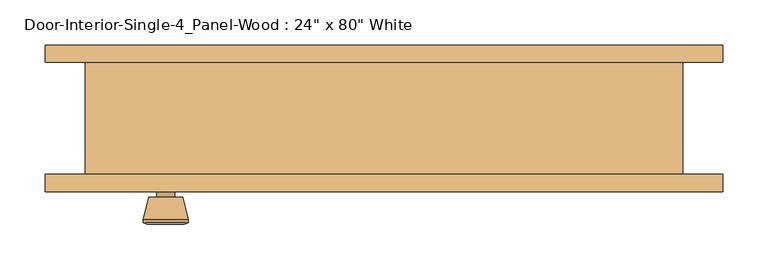
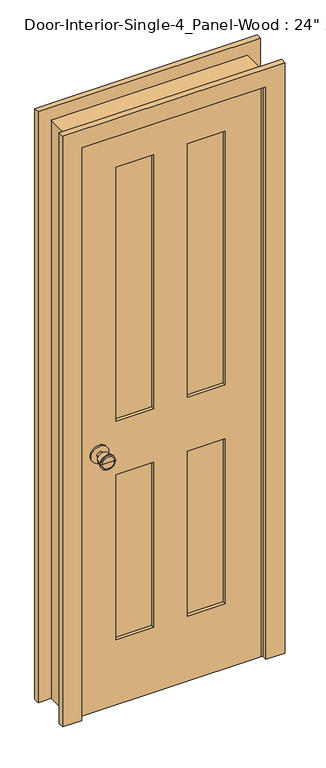
"""IFC4 building model written with IfcOpenShell, lengths in millimetres: door geometry."""

from ifc_helpers import new_model, si_unit, point, frame, frame_2d, origin, place, context, project, spatial, polyline, circle_curve, trimmed, segment, composite_curve, outline, extrude, faceted_brep, source, transform, mapped, element, save
from ifc_brep_helpers import plane_surface, cylinder_surface, revolved_surface, advanced_brep


def door_cd006500(model_context):
    return source(origin(), model_context, "Body", "SolidModel", [
        advanced_brep(
        [(-241.3, -17.8125, 914.4), (-251.3, -17.8125, 914.4), (-231.3, -17.8125, 914.4), (-220.8241324, 31.1875, 914.4), (-261.7758676, 31.1875, 914.4), (-241.3, 31.1875, 914.4), (-216.3, 29.3596319, 914.4), (-266.3, 29.3596319, 914.4), (-216.3, 25.8959537, 914.4), (-266.3, 25.8959537, 914.4), (-222.663764, 1.1875, 914.4), (-259.936236, 1.1875, 914.4), (-231.3, 1.1875, 914.4), (-251.3, 1.1875, 914.4)],
        [
            (0, 1),
            (1, 2, circle_curve(frame((-241.3, -17.8125, 914.4), z_axis=(0.0, -1.0, 0.0), x_axis=(-1.0, 0.0, 0.0)), 10.0)),
            (2, 0),
            (2, 1, circle_curve(frame((-241.3, -17.8125, 914.4), z_axis=(0.0, -1.0, 0.0), x_axis=(-1.0, 0.0, 0.0)), 10.0)),
            (3, 4, circle_curve(frame((-241.3, 31.1875, 914.4), z_axis=(0.0, 1.0, 0.0), x_axis=(-1.0, 0.0, 0.0)), 20.4758676)),
            (4, 5),
            (5, 3),
            (4, 3, circle_curve(frame((-241.3, 31.1875, 914.4), z_axis=(0.0, 1.0, 0.0), x_axis=(-1.0, 0.0, 0.0)), 20.4758676)),
            (6, 7, circle_curve(frame((-241.3, 29.3596319, 914.4), z_axis=(0.0, 1.0, 0.0), x_axis=(-1.0, 0.0, 0.0)), 25.0)),
            (7, 4),
            (3, 6),
            (7, 6, circle_curve(frame((-241.3, 29.3596319, 914.4), z_axis=(0.0, 1.0, 0.0), x_axis=(-1.0, 0.0, 0.0)), 25.0)),
            (8, 9, circle_curve(frame((-241.3, 25.8959537, 914.4), z_axis=(0.0, 1.0, 0.0), x_axis=(-1.0, 0.0, 0.0)), 25.0)),
            (9, 7),
            (6, 8),
            (9, 8, circle_curve(frame((-241.3, 25.8959537, 914.4), z_axis=(0.0, 1.0, 0.0), x_axis=(-1.0, 0.0, 0.0)), 25.0)),
            (10, 11, circle_curve(frame((-241.3, 1.1875, 914.4), z_axis=(0.0, 1.0, 0.0), x_axis=(-1.0, 0.0, 0.0)), 18.636236)),
            (11, 9),
            (8, 10),
            (11, 10, circle_curve(frame((-241.3, 1.1875, 914.4), z_axis=(0.0, 1.0, 0.0), x_axis=(-1.0, 0.0, 0.0)), 18.636236)),
            (12, 13, circle_curve(frame((-241.3, 1.1875, 914.4), z_axis=(0.0, 1.0, 0.0), x_axis=(-1.0, 0.0, 0.0)), 10.0)),
            (13, 11),
            (10, 12),
            (13, 12, circle_curve(frame((-241.3, 1.1875, 914.4), z_axis=(0.0, 1.0, 0.0), x_axis=(-1.0, 0.0, 0.0)), 10.0)),
            (1, 13),
            (12, 2),
        ],
        [
            plane_surface(frame((-241.3, -17.8125, 914.4), z_axis=(0.0, -1.0, 0.0), x_axis=(-1.0, 0.0, 0.0))),
            plane_surface(frame((-241.3, 31.1875, 914.4), z_axis=(0.0, 1.0, 0.0), x_axis=(-1.0, 0.0, 0.0))),
            revolved_surface(polyline([(-261.7758676, 31.1875, 914.4), (-266.3, 29.3596319, 914.4)]), (-241.3, -17.8125, 914.4), (0.0, -1.0, 0.0)),
            cylinder_surface(frame((-241.3, -17.8125, 914.4), z_axis=(0.0, -1.0, 0.0), x_axis=(-1.0, 0.0, 0.0)), 25.0),
            revolved_surface(polyline([(-266.3, 25.8959537, 914.4), (-259.936236, 1.1875, 914.4)]), (-241.3, -17.8125, 914.4), (0.0, -1.0, 0.0)),
            plane_surface(frame((-241.3, 1.1875, 914.4), z_axis=(0.0, -1.0, 0.0), x_axis=(-1.0, 0.0, 0.0))),
            cylinder_surface(frame((-241.3, -17.8125, 914.4), z_axis=(0.0, -1.0, 0.0), x_axis=(-1.0, 0.0, 0.0)), 10.0),
        ],
        [
            (0, [[1, 2, 3]]),
            (0, [[-3, 4, -1]]),
            (1, [[5, 6, 7]]),
            (1, [[8, -7, -6]]),
            (2, [[9, 10, -5, 11]]),
            (2, [[12, -11, -8, -10]]),
            (3, [[13, 14, -9, 15]]),
            (3, [[16, -15, -12, -14]]),
            (4, [[17, 18, -13, 19]]),
            (4, [[20, -19, -16, -18]]),
            (5, [[21, 22, -17, 23]]),
            (5, [[24, -23, -20, -22]]),
            (6, [[-2, 25, -21, 26]]),
            (6, [[-4, -26, -24, -25]]),
        ],
    ),
        extrude(outline(composite_curve([segment(trimmed(circle_curve(frame_2d((914.4, -241.3)), 30.0), [point((914.4, -271.3))], [point((914.4, -211.3))], False, "CARTESIAN"), True, "CONTINUOUS"), segment(trimmed(circle_curve(frame_2d((914.4, -241.3)), 30.0), [point((914.4, -211.3))], [point((914.4, -271.3))], False, "CARTESIAN"), True, "CONTINUOUS")], self_intersect=False)), frame((0.0, -23.8125, 0.0), z_axis=(0.0, 1.0, 0.0), x_axis=(0.0, 0.0, 1.0)), (0.0, 0.0, 1.0), 6.0),
        advanced_brep(
        [(-241.3, -64.7375, 914.4), (-231.3, -64.7375, 914.4), (-251.3, -64.7375, 914.4), (-220.8241324, -113.7375, 914.4), (-241.3, -113.7375, 914.4), (-261.7758676, -113.7375, 914.4), (-216.3, -111.9096319, 914.4), (-266.3, -111.9096319, 914.4), (-216.3, -108.4459537, 914.4), (-266.3, -108.4459537, 914.4), (-222.663764, -83.7375, 914.4), (-259.936236, -83.7375, 914.4), (-231.3, -83.7375, 914.4), (-251.3, -83.7375, 914.4)],
        [
            (0, 1),
            (1, 2, circle_curve(frame((-241.3, -64.7375, 914.4), z_axis=(0.0, 1.0, 0.0), x_axis=(-1.0, 0.0, 0.0)), 10.0)),
            (2, 0),
            (2, 1, circle_curve(frame((-241.3, -64.7375, 914.4), z_axis=(0.0, 1.0, 0.0), x_axis=(-1.0, 0.0, 0.0)), 10.0)),
            (3, 4),
            (4, 5),
            (5, 3, circle_curve(frame((-241.3, -113.7375, 914.4), z_axis=(0.0, -1.0, 0.0), x_axis=(-1.0, 0.0, 0.0)), 20.4758676)),
            (3, 5, circle_curve(frame((-241.3, -113.7375, 914.4), z_axis=(0.0, -1.0, 0.0), x_axis=(-1.0, 0.0, 0.0)), 20.4758676)),
            (6, 3),
            (5, 7),
            (7, 6, circle_curve(frame((-241.3, -111.9096319, 914.4), z_axis=(0.0, -1.0, 0.0), x_axis=(-1.0, 0.0, 0.0)), 25.0)),
            (6, 7, circle_curve(frame((-241.3, -111.9096319, 914.4), z_axis=(0.0, -1.0, 0.0), x_axis=(-1.0, 0.0, 0.0)), 25.0)),
            (8, 6),
            (7, 9),
            (9, 8, circle_curve(frame((-241.3, -108.4459537, 914.4), z_axis=(0.0, -1.0, 0.0), x_axis=(-1.0, 0.0, 0.0)), 25.0)),
            (8, 9, circle_curve(frame((-241.3, -108.4459537, 914.4), z_axis=(0.0, -1.0, 0.0), x_axis=(-1.0, 0.0, 0.0)), 25.0)),
            (10, 8),
            (9, 11),
            (11, 10, circle_curve(frame((-241.3, -83.7375, 914.4), z_axis=(0.0, -1.0, 0.0), x_axis=(-1.0, 0.0, 0.0)), 18.636236)),
            (10, 11, circle_curve(frame((-241.3, -83.7375, 914.4), z_axis=(0.0, -1.0, 0.0), x_axis=(-1.0, 0.0, 0.0)), 18.636236)),
            (12, 10),
            (11, 13),
            (13, 12, circle_curve(frame((-241.3, -83.7375, 914.4), z_axis=(0.0, -1.0, 0.0), x_axis=(-1.0, 0.0, 0.0)), 10.0)),
            (12, 13, circle_curve(frame((-241.3, -83.7375, 914.4), z_axis=(0.0, -1.0, 0.0), x_axis=(-1.0, 0.0, 0.0)), 10.0)),
            (1, 12),
            (13, 2),
        ],
        [
            plane_surface(frame((-241.3, -64.7375, 914.4), z_axis=(0.0, 1.0, 0.0), x_axis=(-1.0, 0.0, 0.0))),
            plane_surface(frame((-241.3, -113.7375, 914.4), z_axis=(0.0, -1.0, 0.0), x_axis=(-1.0, 0.0, 0.0))),
            revolved_surface(polyline([(-261.7758676, -113.7375, 914.4), (-266.3, -111.9096319, 914.4)]), (-241.3, -64.7375, 914.4), (0.0, 1.0, 0.0)),
            cylinder_surface(frame((-241.3, -64.7375, 914.4), z_axis=(0.0, 1.0, 0.0), x_axis=(-1.0, 0.0, 0.0)), 25.0),
            revolved_surface(polyline([(-266.3, -108.4459537, 914.4), (-259.936236, -83.7375, 914.4)]), (-241.3, -64.7375, 914.4), (0.0, 1.0, 0.0)),
            plane_surface(frame((-241.3, -83.7375, 914.4), z_axis=(0.0, 1.0, 0.0), x_axis=(-1.0, 0.0, 0.0))),
            cylinder_surface(frame((-241.3, -64.7375, 914.4), z_axis=(0.0, 1.0, 0.0), x_axis=(-1.0, 0.0, 0.0)), 10.0),
        ],
        [
            (0, [[1, 2, 3]]),
            (0, [[-3, 4, -1]]),
            (1, [[5, 6, 7]]),
            (1, [[-6, -5, 8]]),
            (2, [[9, -7, 10, 11]]),
            (2, [[-10, -8, -9, 12]]),
            (3, [[13, -11, 14, 15]]),
            (3, [[-14, -12, -13, 16]]),
            (4, [[17, -15, 18, 19]]),
            (4, [[-18, -16, -17, 20]]),
            (5, [[21, -19, 22, 23]]),
            (5, [[-22, -20, -21, 24]]),
            (6, [[25, -23, 26, -2]]),
            (6, [[-26, -24, -25, -4]]),
        ],
    ),
        extrude(outline(composite_curve([segment(trimmed(circle_curve(frame_2d((914.4, -241.3)), 30.0), [point((914.4, -271.3))], [point((914.4, -211.3))], False, "CARTESIAN"), True, "CONTINUOUS"), segment(trimmed(circle_curve(frame_2d((914.4, -241.3)), 30.0), [point((914.4, -211.3))], [point((914.4, -271.3))], False, "CARTESIAN"), True, "CONTINUOUS")], self_intersect=False)), frame((0.0, -64.7375, 0.0), z_axis=(0.0, 1.0, 0.0), x_axis=(0.0, 0.0, 1.0)), (0.0, 0.0, 1.0), 6.0),
        extrude(outline(polyline([(184.15, -35.4541667), (184.15, -47.0958333), (57.15, -47.0958333), (57.15, -35.4541667), (184.15, -35.4541667)])), frame((0.0, 0.0, 1009.65), z_axis=(0.0, 0.0, 1.0), x_axis=(1.0, 0.0, 0.0)), (0.0, 0.0, 1.0), 903.2875),
        extrude(outline(polyline([(-57.15, -35.4541667), (-57.15, -47.0958333), (-184.15, -47.0958333), (-184.15, -35.4541667), (-57.15, -35.4541667)])), frame((0.0, 0.0, 1009.65), z_axis=(0.0, 0.0, 1.0), x_axis=(1.0, 0.0, 0.0)), (0.0, 0.0, 1.0), 903.2875),
        extrude(outline(polyline([(184.15, -35.4541667), (184.15, -47.0958333), (57.15, -47.0958333), (57.15, -35.4541667), (184.15, -35.4541667)])), frame((0.0, 0.0, 231.775), z_axis=(0.0, 0.0, 1.0), x_axis=(1.0, 0.0, 0.0)), (0.0, 0.0, 1.0), 587.375),
        extrude(outline(polyline([(-57.15, -35.4541667), (-57.15, -47.0958333), (-184.15, -47.0958333), (-184.15, -35.4541667), (-57.15, -35.4541667)])), frame((0.0, 0.0, 231.775), z_axis=(0.0, 0.0, 1.0), x_axis=(1.0, 0.0, 0.0)), (0.0, 0.0, 1.0), 587.375),
        extrude(outline(polyline([(2032.0, -304.8), (0.0, -304.8), (0.0, 304.8), (2032.0, 304.8), (2032.0, -304.8)]), holes=[polyline([(1912.9375, 57.15), (1912.9375, 184.15), (1009.65, 184.15), (1009.65, 57.15), (1912.9375, 57.15)]), polyline([(1009.65, -57.15), (1009.65, -184.15), (1912.9375, -184.15), (1912.9375, -57.15), (1009.65, -57.15)]), polyline([(819.15, 57.15), (819.15, 184.15), (231.775, 184.15), (231.775, 57.15), (819.15, 57.15)]), polyline([(231.775, -57.15), (231.775, -184.15), (819.15, -184.15), (819.15, -57.15), (231.775, -57.15)])]), frame((0.0, -58.7375, 0.0), z_axis=(0.0, 1.0, 0.0), x_axis=(0.0, 0.0, 1.0)), (0.0, 0.0, 1.0), 34.925),
        faceted_brep([(330.2, -58.7375, 0.0), (304.8, -58.7375, 0.0), (304.8, -23.8125, 0.0), (292.1, -23.8125, 0.0), (292.1, 11.1125, 0.0), (304.8, 11.1125, 0.0), (304.8, 65.0875, 0.0), (330.2, 65.0875, 0.0), (330.2, 65.0875, 2057.4), (330.2, -58.7375, 2057.4), (304.8, 65.0875, 2032.0), (-304.8, 65.0875, 2032.0), (-304.8, 65.0875, 0.0), (-330.2, 65.0875, 0.0), (-330.2, 65.0875, 2057.4), (304.8, 11.1125, 2032.0), (292.1, 11.1125, 2019.3), (-292.1, 11.1125, 2019.3), (-292.1, 11.1125, 0.0), (-304.8, 11.1125, 0.0), (-304.8, 11.1125, 2032.0), (292.1, -23.8125, 2019.3), (304.8, -23.8125, 2032.0), (-304.8, -23.8125, 2032.0), (-304.8, -23.8125, 0.0), (-292.1, -23.8125, 0.0), (-292.1, -23.8125, 2019.3), (304.8, -58.7375, 2032.0), (-330.2, -58.7375, 2057.4), (-330.2, -58.7375, 0.0), (-304.8, -58.7375, 0.0), (-304.8, -58.7375, 2032.0)], [[[0, 1, 2, 3, 4, 5, 6, 7]], [[7, 8, 9, 0]], [[6, 10, 11, 12, 13, 14, 8, 7]], [[5, 15, 10, 6]], [[4, 16, 17, 18, 19, 20, 15, 5]], [[3, 21, 16, 4]], [[2, 22, 23, 24, 25, 26, 21, 3]], [[1, 27, 22, 2]], [[0, 9, 28, 29, 30, 31, 27, 1]], [[8, 14, 28, 9]], [[15, 20, 11, 10]], [[21, 26, 17, 16]], [[27, 31, 23, 22]], [[29, 13, 12, 19, 18, 25, 24, 30]], [[14, 13, 29, 28]], [[20, 19, 12, 11]], [[26, 25, 18, 17]], [[31, 30, 24, 23]]]),
        extrude(outline(polyline([(0.0, 374.65), (2101.85, 374.65), (2101.85, -374.65), (0.0, -374.65), (0.0, -311.15), (2038.35, -311.15), (2038.35, 311.15), (0.0, 311.15), (0.0, 374.65)])), frame((0.0, 65.0875, 0.0), z_axis=(0.0, 1.0, 0.0), x_axis=(0.0, 0.0, 1.0)), (0.0, 0.0, 1.0), 19.05),
        extrude(outline(polyline([(0.0, 374.65), (2101.85, 374.65), (2101.85, -374.65), (0.0, -374.65), (0.0, -311.15), (2038.35, -311.15), (2038.35, 311.15), (0.0, 311.15), (0.0, 374.65)])), frame((0.0, -77.7875, 0.0), z_axis=(0.0, 1.0, 0.0), x_axis=(0.0, 0.0, 1.0)), (0.0, 0.0, 1.0), 19.05),
    ])


if __name__ == "__main__":
    model = new_model("IFC4")
    model_context = context("Model", 3, world=origin())
    ifc_project = project(units=[si_unit("LENGTHUNIT", "METRE", prefix="MILLI")], contexts=[model_context])
    site = spatial("IfcSite", under=ifc_project)
    building = spatial("IfcBuilding", under=site)
    placement = place(None, origin())
    door_shape = door_cd006500(model_context)
    element("IfcDoor", 1, ObjectType="Door-Interior-Single-4_Panel-Wood : 24\" x 80\" White", at=placement, inside=building, context=model_context, shape_type="MappedRepresentation", body=[
        mapped(door_shape, transform((0.0, 0.0, 0.0), x_axis=(1.0, 0.0, 0.0), y_axis=(0.0, 1.0, 0.0), z_axis=(0.0, 0.0, 1.0))),
    ])
    save(model, "model.ifc")

# Revit data of these elements
# Type "Door-Interior-Single-4_Panel-Wood : 24\" x 80\" White"
#   Type Mark = "49"
#   COBie.Type.CreatedBy = "doug.wood@us.ibm.com"
#   COBie.Type.CreatedOn = "2016-04-14T02:07:24"
#   COBie.Type.Name = "Doors_Door-Interior-Single-4_Panel-Wood_24\" x 80\" White_49"
#   COBie.Type.Category = "23-30 10 00 : Doors"
#   COBie.Type.Description = "Door-Interior-Single-4_Panel-Wood_24\" x 80\" White"
#   COBie.Type.Manufacturer = ""
#   COBie.Type.ModelNumber = ""
#   Assembly Code = "C1020300"
#   Analytic Construction = "Wooden"
#   COBie.Type.ReplacementCost = 0
#   Top Rail = 0' - 4 11/16"
#   Thickness = 0' - 1 3/8"
#   Thermal Resistance (R) = 0.455703 (m²·K)/W
#   Swing Angle [instance default] = 90.00°
#   Stiles = 0' - 4 3/4"
#   Rough Width = 2' - 2"
#   Rough Height = 6' - 9"
#   Mullion = 0' - 4 1/2"
#   Lock Rail = 0' - 7 1/2"
#   Height = 6' - 8"
#   Width = 2' - 0"
#   Heat Transfer Coefficient (U) = 2.19465 W/(m²·K)
#   Bottom Rail = 0' - 9 1/8"
#   COBie.Type = no
#   Trim Material = Trim - White
#   Panel Material = Door - Panel - White
#   Frame Material = Door - Panel - White
#   Door Handle Material = ARCAT - Metal - Brass, Polished
#   Visual Light Transmittance = 0
#   Solar Heat Gain Coefficient = 0
#   Wall Closure = (empty or 0)
#   Function = (empty or 0)
# Element 1 (IfcDoor, "Door-Interior-Single-4_Panel-Wood : 24\" x 80\" White")
#   Materials on its faces: "Door - Panel - White", "ARCAT - Metal - Brass, Polished", "Trim - White"
# Materials
#   "Trim - White": class "Wood", colour RGB 255 255 255, transparency 0, Cost = 0
#   "Door - Panel - White": class "Wood", colour RGB 255 255 255, transparency 0, Cost = 0
#   "ARCAT - Metal - Brass, Polished": class "Unassigned", colour RGB 246 240 166, transparency 0, Keynote = "05050", Model = "Generic", Manufacturer = "Generic", Description = "Steel, Chrome Plated"
